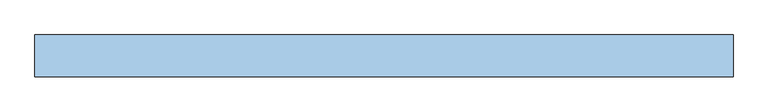
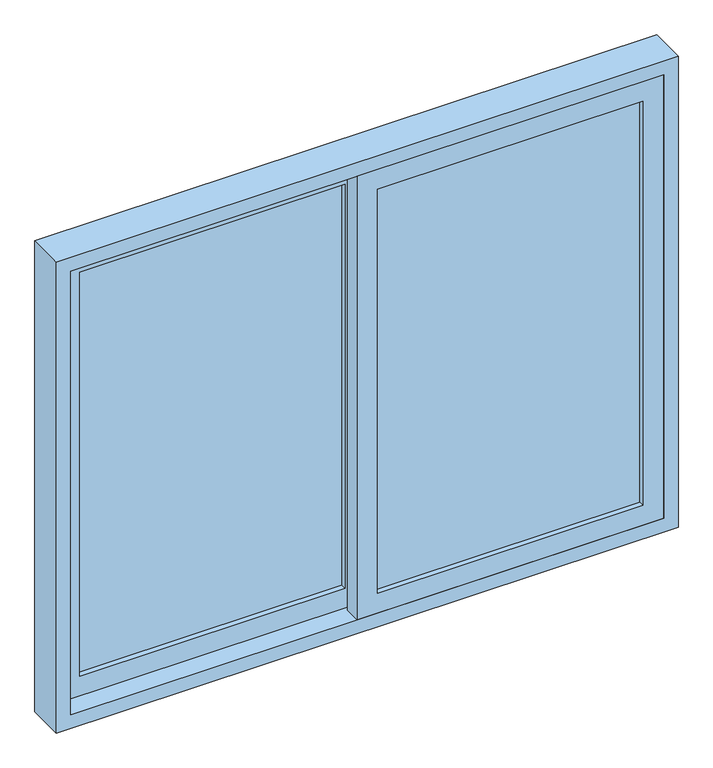
"""IFC4 building model written with IfcOpenShell, lengths in millimetres: window geometry, Janela de correr - 2 Painéis : Janela de correr - 2 Painéis 1,50m."""

from ifc_helpers import new_model, si_unit, frame, origin, place, context, project, spatial, polyline, outline, extrude, source, transform, mapped, element, save


def window_4c519cc2(model_context):
    return source(origin(), model_context, "Body", "SweptSolid", [
        extrude(outline(polyline([(1815.0, -25.0), (685.0, -25.0), (685.0, 715.0), (1815.0, 715.0), (1815.0, -25.0)]), holes=[polyline([(735.0, 25.0), (1765.0, 25.0), (1765.0, 665.0), (735.0, 665.0), (735.0, 25.0)])]), frame((0.0, -20.0, 0.0), z_axis=(0.0, 1.0, 0.0), x_axis=(0.0, 0.0, 1.0)), (0.0, 0.0, 1.0), 40.0),
        extrude(outline(polyline([(685.0, 25.0), (1815.0, 25.0), (1815.0, -715.0), (685.0, -715.0), (685.0, 25.0)]), holes=[polyline([(1765.0, -25.0), (735.0, -25.0), (735.0, -665.0), (1765.0, -665.0), (1765.0, -25.0)])]), frame((0.0, 30.0, 0.0), z_axis=(0.0, 1.0, 0.0), x_axis=(0.0, 0.0, 1.0)), (0.0, 0.0, 1.0), 40.0),
        extrude(outline(polyline([(650.0, 750.0), (1850.0, 750.0), (1850.0, -750.0), (650.0, -750.0), (650.0, 750.0)]), holes=[polyline([(1815.0, 715.0), (685.0, 715.0), (685.0, -715.0), (1815.0, -715.0), (1815.0, 715.0)])]), frame((0.0, -20.0, 0.0), z_axis=(0.0, 1.0, 0.0), x_axis=(0.0, 0.0, 1.0)), (0.0, 0.0, 1.0), 90.0),
        extrude(outline(polyline([(25.0, -7.0), (25.0, 7.0), (665.0, 7.0), (665.0, -7.0), (25.0, -7.0)])), frame((0.0, 0.0, 735.0), z_axis=(0.0, 0.0, 1.0), x_axis=(1.0, 0.0, 0.0)), (0.0, 0.0, 1.0), 1030.0),
        extrude(outline(polyline([(-665.0, 43.0), (-665.0, 57.0), (-25.0, 57.0), (-25.0, 43.0), (-665.0, 43.0)])), frame((0.0, 0.0, 735.0), z_axis=(0.0, 0.0, 1.0), x_axis=(1.0, 0.0, 0.0)), (0.0, 0.0, 1.0), 1030.0),
    ])


if __name__ == "__main__":
    model = new_model("IFC4")
    model_context = context("Model", 3, world=origin())
    ifc_project = project(units=[si_unit("LENGTHUNIT", "METRE", prefix="MILLI")], contexts=[model_context])
    site = spatial("IfcSite", under=ifc_project)
    building = spatial("IfcBuilding", under=site)
    placement = place(None, origin())
    window_shape = window_4c519cc2(model_context)
    element("IfcWindow", 1, ObjectType="Janela de correr - 2 Painéis : Janela de correr - 2 Painéis 1,50m", at=placement, inside=building, context=model_context, shape_type="MappedRepresentation", body=[
        mapped(window_shape, transform((0.0, 0.0, 0.0), x_axis=(1.0, 0.0, 0.0), y_axis=(0.0, 1.0, 0.0), z_axis=(0.0, 0.0, 1.0))),
    ])
    save(model, "model.ifc")

# Revit data of these elements
# Type "Janela de correr - 2 Painéis : Janela de correr - 2 Painéis 1,50m"
#   Type Mark = "EF29"
#   Construction Type Id = "GSP4R"
#   Analytic Construction = "Vidraça única Pilkington 1/8 pol"
#   Visual Light Transmittance = 0.9
#   Solar Heat Gain Coefficient = 0.78
#   Rough Width = 1.500 m
#   Rough Height = 1.200 m
#   Largura da moldura do painel = 0.050 m
#   Espessura da moldura do painel = 0.040 m
#   Height = 1.200 m
#   Heat Transfer Coefficient (U) = 3.6886 W/(m²·K)
#   Largura da estrutura = 0.035 m
#   Espessura da moldura = 0.090 m
#   Altura-padrão do peitoril = 0.650 m
#   Width = 1.500 m
#   Define Thermal Properties by = 1
#   Vidro = none
#   Material da moldura = none
#   Wall Closure = (empty or 0)
# Element 1 (IfcWindow, "Janela de correr - 2 Painéis : Janela de correr - 2 Painéis 1,50m")
#   Materials on its faces: "Glass"
# Materials
#   "Glass": class "Glass", colour RGB 0 128 192, transparency 0.75, Description = "Soda Lime Glass", Cost = 0
